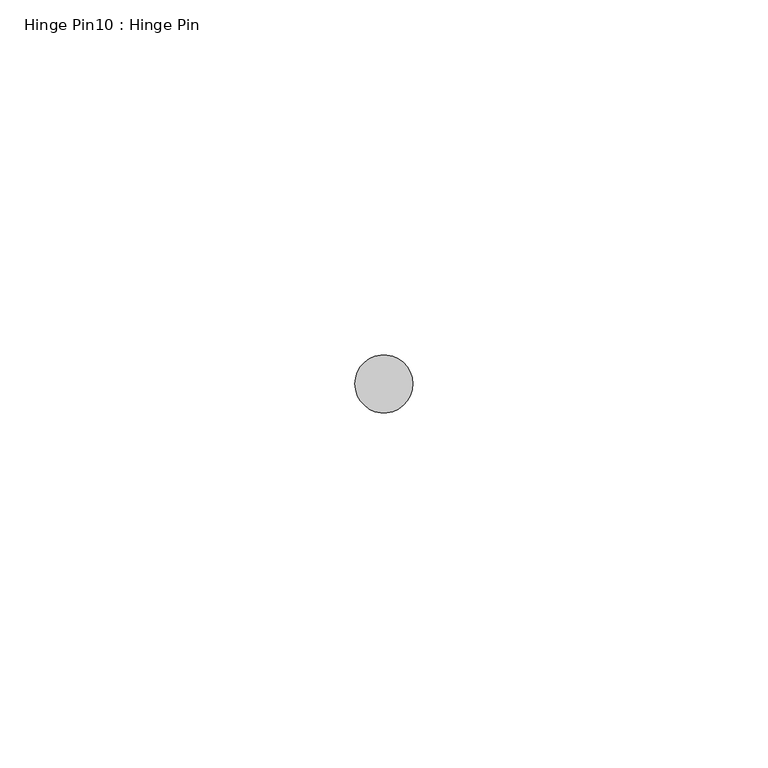
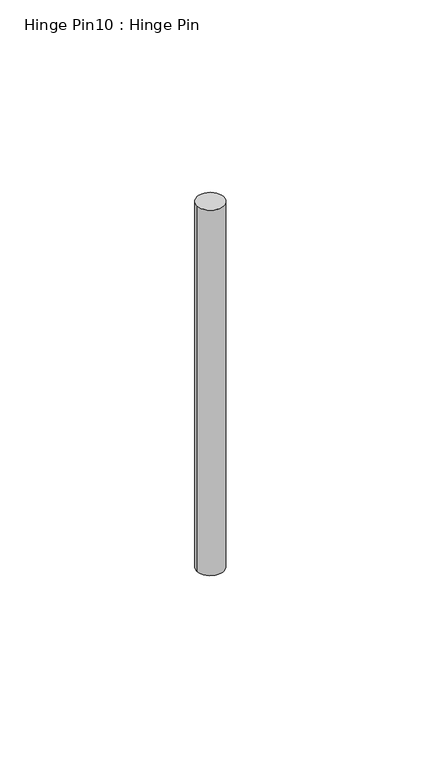
"""IFC4 building model written with IfcOpenShell, lengths in millimetres: proxy geometry, Hinge Pin10 : Hinge Pin."""

import ifcopenshell
import ifcopenshell.guid

model = None  # the IFC model being written
_history = None  # IfcOwnerHistory: only IFC2X3 demands one
_inside = {}  # id of a spatial element -> (the spatial element, [elements in it])
_under = {}  # id of a project, library or spatial element -> (it, [spatial elements below it])
_declared = {}  # id of a project -> (the project, [libraries it declares])
_typed = {}  # id of a type object -> (the type object, [elements of that type])
_made_of = {}  # id of a material, layer set ... -> (it, [elements and type objects made of it])


def new_model(schema):
    """Start an empty IFC model of exactly this schema.

    Asked for "IFC4X3", IfcOpenShell would pick the latest addendum, in which some entities
    have other attributes; the version numbers below select the first issue.
    IFC2X3 requires an IfcOwnerHistory on every rooted entity: one is made here for all.
    """
    global model, _history
    if schema == "IFC4X3":
        model = ifcopenshell.file(schema_version=(4, 3, 0, 0))
    else:
        model = ifcopenshell.file(schema=schema)
    _inside.clear()
    _under.clear()
    _declared.clear()
    _typed.clear()
    _made_of.clear()
    _history = None
    if model.schema == "IFC2X3":
        org = make("IfcOrganization", Name="unknown")
        user = make(
            "IfcPersonAndOrganization",
            ThePerson=make("IfcPerson", FamilyName="unknown"),
            TheOrganization=org,
        )
        app = make(
            "IfcApplication",
            ApplicationDeveloper=org,
            Version="unknown",
            ApplicationFullName="unknown",
            ApplicationIdentifier="unknown",
        )
        _history = make(
            "IfcOwnerHistory",
            OwningUser=user,
            OwningApplication=app,
            ChangeAction="ADDED",
            CreationDate=0,
        )
    return model


def make(cls, **values):
    """One entity of the class cls with the attributes given. An attribute that is None is left unset."""
    return model.create_entity(
        cls, **{name: value for name, value in values.items() if value is not None}
    )


def rooted(cls, **values):
    """An entity with a GlobalId (a new one), such as an element, a storey or a relation."""
    return make(cls, GlobalId=ifcopenshell.guid.new(), OwnerHistory=_history, **values)


def si_unit(unit_type, name, prefix=None):
    """IfcSIUnit, for example si_unit("LENGTHUNIT", "METRE", prefix="MILLI")."""
    return make("IfcSIUnit", UnitType=unit_type, Prefix=prefix, Name=name)


def assignment(units):
    """IfcUnitAssignment: the units of a project."""
    return None if units is None else make("IfcUnitAssignment", Units=units)


def point(xyz):
    """IfcCartesianPoint."""
    return None if xyz is None else make("IfcCartesianPoint", Coordinates=xyz)


def direction(xyz):
    """IfcDirection."""
    return None if xyz is None else make("IfcDirection", DirectionRatios=xyz)


def frame(location, z_axis=None, x_axis=None):
    """IfcAxis2Placement3D, a coordinate frame: its origin and axes. An axis left out is left unset."""
    return make(
        "IfcAxis2Placement3D",
        Location=point(location),
        Axis=direction(z_axis),
        RefDirection=direction(x_axis),
    )


def frame_2d(location, x_axis=None):
    """IfcAxis2Placement2D, a coordinate frame in the plane: its origin and x axis."""
    return make(
        "IfcAxis2Placement2D", Location=point(location), RefDirection=direction(x_axis)
    )


def origin():
    """The frame at (0, 0, 0) with its axes left unset."""
    return frame((0.0, 0.0, 0.0))


def place(relative_to, where):
    """IfcLocalPlacement: puts the frame where relative to a parent placement (None: the world)."""
    return make(
        "IfcLocalPlacement", PlacementRelTo=relative_to, RelativePlacement=where
    )


def context(
    kind, dimensions, precision=None, world=None, true_north=None, identifier=None
):
    """IfcGeometricRepresentationContext, for example the 3D "Model" context."""
    return make(
        "IfcGeometricRepresentationContext",
        ContextIdentifier=identifier,
        ContextType=kind,
        CoordinateSpaceDimension=dimensions,
        Precision=precision,
        WorldCoordinateSystem=world,
        TrueNorth=true_north,
    )


def project(units=None, contexts=None):
    """IfcProject with its units and contexts."""
    return rooted(
        "IfcProject",
        Name="project",
        RepresentationContexts=contexts,
        UnitsInContext=assignment(units),
    )


def spatial(cls, under=None, at=None, **own):
    """A site, building, storey or space (cls), placed at a placement, below another one or the project."""
    s = rooted(cls, ObjectPlacement=at, **own)
    if under is not None:
        _under.setdefault(under.id(), (under, []))[1].append(s)
    return s


def circle_curve(where, radius):
    """IfcCircle in the frame where."""
    return make("IfcCircle", Position=where, Radius=radius)


def trimmed(basis, trim1, trim2, sense, master):
    """IfcTrimmedCurve: the piece of a basis curve between two trims."""
    return make(
        "IfcTrimmedCurve",
        BasisCurve=basis,
        Trim1=trim1,
        Trim2=trim2,
        SenseAgreement=sense,
        MasterRepresentation=master,
    )


def segment(curve, same_sense, transition):
    """IfcCompositeCurveSegment."""
    return make(
        "IfcCompositeCurveSegment",
        Transition=transition,
        SameSense=same_sense,
        ParentCurve=curve,
    )


def composite_curve(segments, self_intersect=None):
    """IfcCompositeCurve: segments joined end to end."""
    return make("IfcCompositeCurve", Segments=segments, SelfIntersect=self_intersect)


def outline(outer, holes=None, kind="AREA"):
    """IfcArbitraryClosedProfileDef: a profile drawn as a closed curve; with holes, ...WithVoids."""
    if holes is None:
        return make("IfcArbitraryClosedProfileDef", ProfileType=kind, OuterCurve=outer)
    return make(
        "IfcArbitraryProfileDefWithVoids",
        ProfileType=kind,
        OuterCurve=outer,
        InnerCurves=holes,
    )


def extrude(swept, where, along, depth):
    """IfcExtrudedAreaSolid: the profile swept, set in the frame where, extruded along a direction by depth."""
    return make(
        "IfcExtrudedAreaSolid",
        SweptArea=swept,
        Position=where,
        ExtrudedDirection=direction(along),
        Depth=depth,
    )


def shape(context_of_items, identifier, shape_type, items):
    """IfcShapeRepresentation: the items that make up one representation, for example the "Body"."""
    return make(
        "IfcShapeRepresentation",
        ContextOfItems=context_of_items,
        RepresentationIdentifier=identifier,
        RepresentationType=shape_type,
        Items=items,
    )


def source(mapping_origin, context_of_items, identifier, shape_type, items):
    """IfcRepresentationMap: a shape defined once, which mapped items show again and again."""
    return make(
        "IfcRepresentationMap",
        MappingOrigin=mapping_origin,
        MappedRepresentation=shape(context_of_items, identifier, shape_type, items),
    )


def transform(
    local_origin,
    x_axis=None,
    y_axis=None,
    z_axis=None,
    scale=None,
    scale2=None,
    scale3=None,
    uniform=True,
):
    """IfcCartesianTransformationOperator3D, or its non-uniform kind. x_axis, y_axis, z_axis: its Axis1, 2, 3."""
    if uniform:
        return make(
            "IfcCartesianTransformationOperator3D",
            Axis1=direction(x_axis),
            Axis2=direction(y_axis),
            LocalOrigin=point(local_origin),
            Scale=scale,
            Axis3=direction(z_axis),
        )
    return make(
        "IfcCartesianTransformationOperator3DnonUniform",
        Axis1=direction(x_axis),
        Axis2=direction(y_axis),
        LocalOrigin=point(local_origin),
        Scale=scale,
        Axis3=direction(z_axis),
        Scale2=scale2,
        Scale3=scale3,
    )


def mapped(mapping_source, mapping_target):
    """IfcMappedItem: shows the shape of a source again, moved by a transform."""
    return make(
        "IfcMappedItem", MappingSource=mapping_source, MappingTarget=mapping_target
    )


def made_of(thing, what):
    """Note that an element or type object is made of a material, layer set ...; save() writes the relation."""
    if what is not None:
        _made_of.setdefault(what.id(), (what, []))[1].append(thing)
    return thing


def element(
    cls,
    number,
    at=None,
    inside=None,
    cuts=None,
    type_object=None,
    material=None,
    context=None,
    identifier="Body",
    shape_type=None,
    held_by="IfcProductDefinitionShape",
    body=None,
    shapes=None,
    **own,
):
    """One element of the class cls, such as IfcWall. Its Tag is "e" and its number.

    at: its placement. inside: the storey or other place that contains it. cuts: it is an
    opening in that element (IfcRelVoidsElement). A single representation is given by context,
    identifier, shape_type and body (its items); several are given by shapes. held_by: the class
    of the entity that holds the representations. save() writes the other relations.
    """
    e = rooted(cls, Tag="e%d" % number, ObjectPlacement=at, **own)
    if body is not None:
        shapes = [shape(context, identifier, shape_type, body)]
    if shapes is not None:
        e.Representation = make(held_by, Representations=shapes)
    if inside is not None:
        _inside.setdefault(inside.id(), (inside, []))[1].append(e)
    if cuts is not None:
        rooted(
            "IfcRelVoidsElement", RelatingBuildingElement=cuts, RelatedOpeningElement=e
        )
    if type_object is not None:
        _typed.setdefault(type_object.id(), (type_object, []))[1].append(e)
    return made_of(e, material)


def aggregate(whole, parts):
    """IfcRelAggregates: a whole, such as a stair, and the parts it consists of."""
    return rooted("IfcRelAggregates", RelatingObject=whole, RelatedObjects=parts)


def save(model, path):
    """Write the relations noted so far, then the file.

    IfcRelAggregates (storeys below a building ...), IfcRelContainedInSpatialStructure (elements
    in a storey), IfcRelDefinesByType, IfcRelAssociatesMaterial and IfcRelDeclares: one each for
    every whole, place, type object, material and project.
    """
    for whole, parts in _under.values():
        aggregate(whole, parts)
    for where, things in _inside.values():
        rooted(
            "IfcRelContainedInSpatialStructure",
            RelatedElements=things,
            RelatingStructure=where,
        )
    for kind, things in _typed.values():
        rooted("IfcRelDefinesByType", RelatedObjects=things, RelatingType=kind)
    for what, things in _made_of.values():
        rooted("IfcRelAssociatesMaterial", RelatedObjects=things, RelatingMaterial=what)
    for by, libraries in _declared.values():
        rooted("IfcRelDeclares", RelatingContext=by, RelatedDefinitions=libraries)
    model.write(path)


def hinge_pin10_hinge_pin_b100999e(model_context):
    return source(origin(), model_context, "Body", "SweptSolid", [
        extrude(outline(composite_curve([segment(trimmed(circle_curve(frame_2d((587319.1320739, -536310.3652841)), 4.0894), [point((587315.0426739, -536310.3652841))], [point((587323.2214739, -536310.3652841))], False, "CARTESIAN"), True, "CONTINUOUS"), segment(trimmed(circle_curve(frame_2d((587319.1320739, -536310.3652841)), 4.0894), [point((587323.2214739, -536310.3652841))], [point((587315.0426739, -536310.3652841))], False, "CARTESIAN"), True, "CONTINUOUS")], self_intersect=False)), frame((0.0, 0.0, 1941.3140625), z_axis=(0.0, 0.0, 1.0), x_axis=(1.0, 0.0, 0.0)), (0.0, 0.0, 1.0), 117.871875),
    ])


if __name__ == "__main__":
    model = new_model("IFC4")
    model_context = context("Model", 3, world=origin())
    ifc_project = project(units=[si_unit("LENGTHUNIT", "METRE", prefix="MILLI")], contexts=[model_context])
    site = spatial("IfcSite", under=ifc_project)
    building = spatial("IfcBuilding", under=site)
    placement = place(None, origin())
    hinge_pin10_hinge_pin_shape = hinge_pin10_hinge_pin_b100999e(model_context)
    element("IfcBuildingElementProxy", 1, Name="Hinge Pin10 : Hinge Pin", ObjectType="Hinge Pin10 : Hinge Pin", at=placement, inside=building, context=model_context, shape_type="MappedRepresentation", body=[
        mapped(hinge_pin10_hinge_pin_shape, transform((0.0, 0.0, 0.0), x_axis=(1.0, 0.0, 0.0), y_axis=(0.0, 1.0, 0.0), z_axis=(0.0, 0.0, 1.0))),
    ])
    save(model, "model.ifc")

# Revit data of these elements
# Element 1 (IfcBuildingElementProxy, "Hinge Pin10 : Hinge Pin")
#   Materials on its faces: "6\"X6\" WELD-ON STL BUTT HINGE"
# Materials
#   "6\"X6\" WELD-ON STL BUTT HINGE": class "Metal", colour RGB 189 187 185, transparency 0, Description = "Carbon steel", Cost = 0
